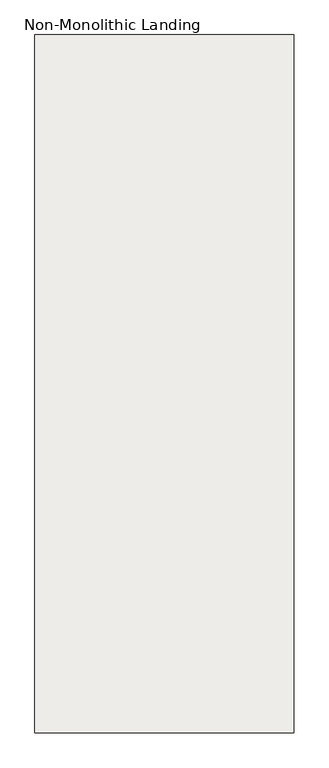
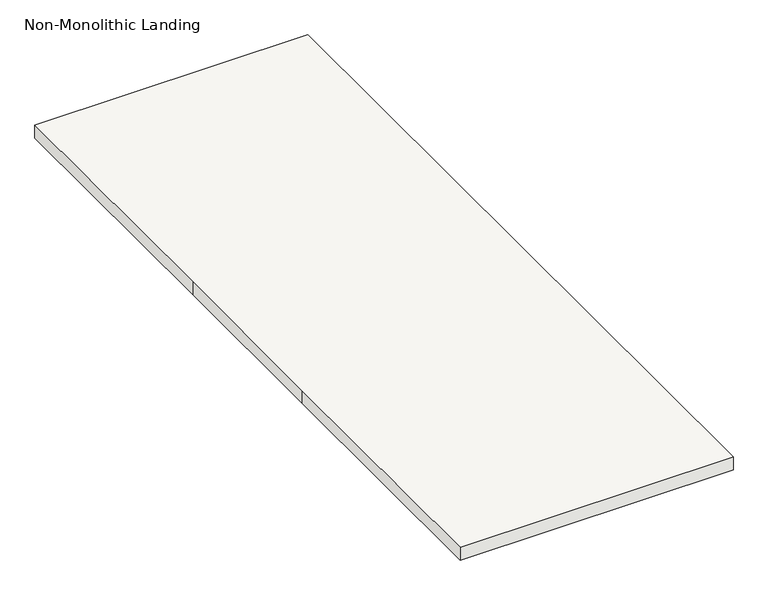
"""IFC4 building model written with IfcOpenShell, lengths in millimetres: slab geometry, Non-Monolithic Landing."""

from ifc_helpers import new_model, si_unit, frame, origin, place, context, project, spatial, polyline, outline, extrude, source, transform, mapped, element, save


def non_monolithic_landing_4132aadd(model_context):
    return source(origin(), model_context, "Body", "SweptSolid", [
        extrude(outline(polyline([(30694.1667192, -3197.3716232), (30694.1667192, -2501.242277), (30694.1667192, -1501.242277), (31694.1667192, -1501.242277), (31694.1667192, -4197.3716232), (30694.1667192, -4197.3716232), (30694.1667192, -3197.3716232)])), frame((0.0, 0.0, 1714.7058824), z_axis=(0.0, 0.0, 1.0), x_axis=(1.0, 0.0, 0.0)), (0.0, 0.0, 1.0), 50.0),
    ])


if __name__ == "__main__":
    model = new_model("IFC4")
    model_context = context("Model", 3, world=origin())
    ifc_project = project(units=[si_unit("LENGTHUNIT", "METRE", prefix="MILLI")], contexts=[model_context])
    site = spatial("IfcSite", under=ifc_project)
    building = spatial("IfcBuilding", under=site)
    placement = place(None, origin())
    non_monolithic_landing_shape = non_monolithic_landing_4132aadd(model_context)
    element("IfcSlab", 1, ObjectType="Non-Monolithic Landing", at=placement, inside=building, context=model_context, shape_type="MappedRepresentation", body=[
        mapped(non_monolithic_landing_shape, transform((0.0, 0.0, 0.0), x_axis=(1.0, 0.0, 0.0), y_axis=(0.0, 1.0, 0.0), z_axis=(0.0, 0.0, 1.0))),
    ])
    save(model, "model.ifc")
